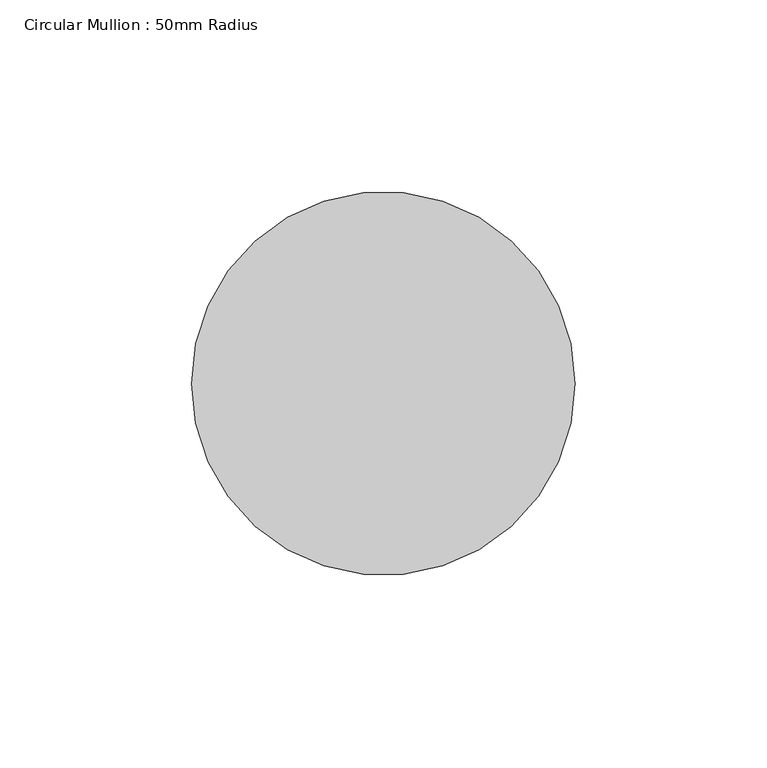
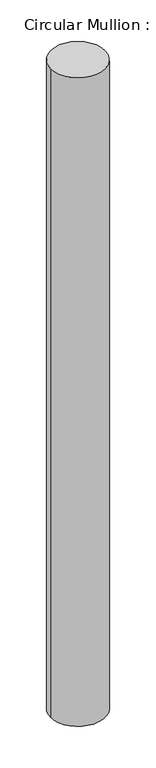
"""IFC4 building model written with IfcOpenShell, lengths in millimetres: member geometry, Circular Mullion : 50mm Radius."""

from ifc_helpers import new_model, si_unit, point, frame, origin, origin_2d, place, context, project, spatial, circle_curve, trimmed, segment, composite_curve, outline, extrude, source, transform, mapped, element, save


def circular_mullion_50mm_radius_17a5a7eb(model_context):
    return source(origin(), model_context, "Body", "SweptSolid", [
        extrude(outline(composite_curve([segment(trimmed(circle_curve(origin_2d(), 50.0), [point((50.0, 0.0))], [point((-50.0, 0.0))], False, "CARTESIAN"), True, "CONTINUOUS"), segment(trimmed(circle_curve(origin_2d(), 50.0), [point((-50.0, 0.0))], [point((50.0, 0.0))], False, "CARTESIAN"), True, "CONTINUOUS")], self_intersect=False)), frame((0.0, 0.0, -1253.8354574), z_axis=(0.0, 0.0, 1.0), x_axis=(1.0, 0.0, 0.0)), (0.0, 0.0, 1.0), 1253.8354574),
    ])


if __name__ == "__main__":
    model = new_model("IFC4")
    model_context = context("Model", 3, world=origin())
    ifc_project = project(units=[si_unit("LENGTHUNIT", "METRE", prefix="MILLI")], contexts=[model_context])
    site = spatial("IfcSite", under=ifc_project)
    building = spatial("IfcBuilding", under=site)
    placement = place(None, origin())
    circular_mullion_50mm_radius_shape = circular_mullion_50mm_radius_17a5a7eb(model_context)
    element("IfcMember", 1, ObjectType="Circular Mullion : 50mm Radius", at=placement, inside=building, context=model_context, shape_type="MappedRepresentation", body=[
        mapped(circular_mullion_50mm_radius_shape, transform((0.0, 0.0, 0.0), x_axis=(1.0, 0.0, 0.0), y_axis=(0.0, 1.0, 0.0), z_axis=(0.0, 0.0, 1.0))),
    ])
    save(model, "model.ifc")

# Revit data of these elements
# Type "Circular Mullion : 50mm Radius"
#   built-in parameter 1007350 = 0.164042 (stored number, unit not read)
# Element 1 (IfcMember, "Circular Mullion : 50mm Radius")
#   Materials on its faces: "Aluminium"
# Materials
#   "Aluminium": class "Metal", colour RGB 247 247 247, transparency 0, Description = "Aluminium 6061", Cost = 0
